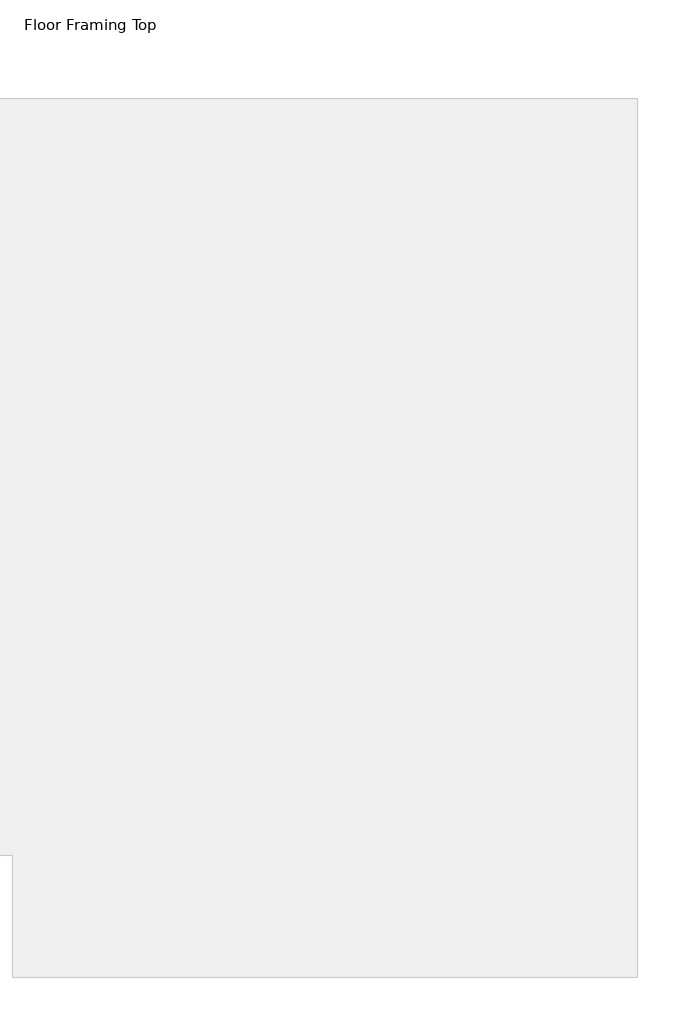
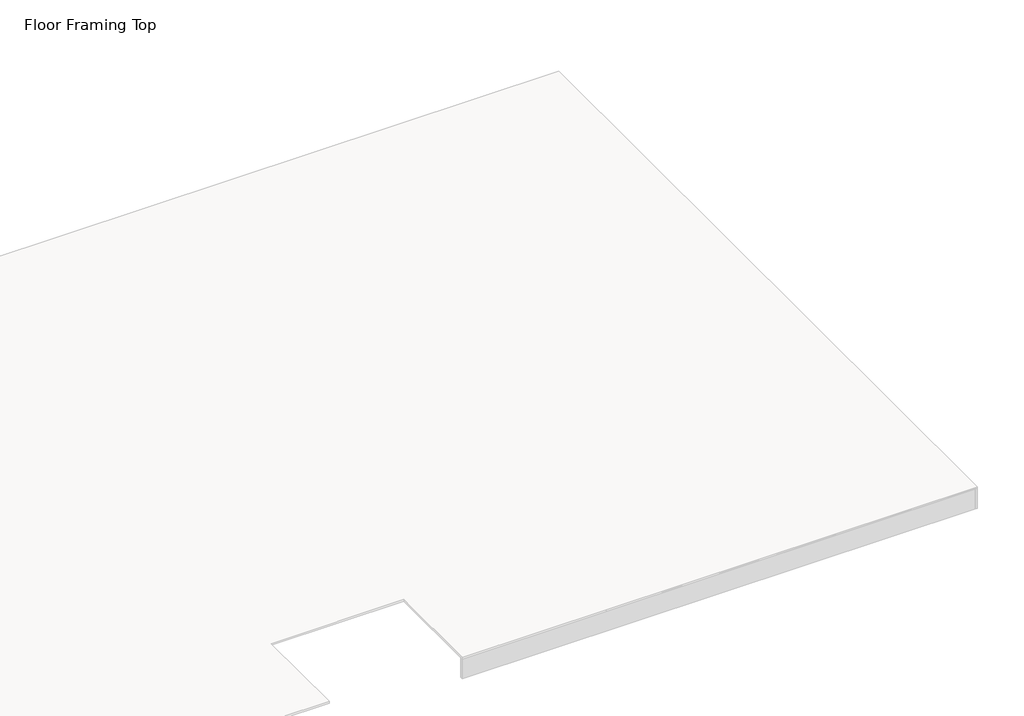
# One storey, part 3 of 4: 17 beams.
"""IFC4 building model written with IfcOpenShell, lengths in millimetres."""

from ifc_helpers import new_model, si_unit, frame, origin, place, context, project, spatial, polyline, outline, extrude, element, save

model = new_model("IFC4")

# Units and contexts
model_context = context("Model", 3, world=origin())
ifc_project = project(units=[si_unit("LENGTHUNIT", "METRE", prefix="MILLI")], contexts=[model_context])

# Site, building, storey
site = spatial("IfcSite", under=ifc_project)
building = spatial("IfcBuilding", under=site)
storey = spatial("IfcBuildingStorey", under=building, Name="Floor Framing Top", Elevation=0.0)

# Beams
placement = place(None, origin())
element("IfcBeam", 1, ObjectType="Plywood Web Joist : 11 7/8 TJI 150", at=placement, inside=storey, context=model_context, shape_type="SweptSolid", body=[
    extrude(outline(polyline([(12853.5472749, -5717.8040947), (12844.0222749, -5717.8040947), (12844.0222749, 4456.4834053), (12853.5472749, 4456.4834053), (12853.5472749, -5717.8040947)])), frame((0.0, 0.0, -269.1410374), z_axis=(0.0, 0.0, 1.0), x_axis=(1.0, 0.0, 0.0)), (0.0, 0.0, 1.0), 237.3910374),
    extrude(outline(polyline([(12844.0222749, -663.2040947), (12844.0222749, 4456.4834053), (12853.5472749, 4456.4834053), (12853.5472749, -663.2040947), (12844.0222749, -663.2040947)])), frame((0.0, 0.0, -269.1410374), z_axis=(0.0, 0.0, 1.0), x_axis=(1.0, 0.0, 0.0)), (0.0, 0.0, 1.0), 237.3910374),
    extrude(outline(polyline([(0.0, 12829.7347749), (-38.1, 12829.7347749), (-38.1, 12844.0222749), (-31.75, 12844.0222749), (-31.75, 12853.5472749), (-38.1, 12853.5472749), (-38.1, 12867.8347749), (0.0, 12867.8347749), (0.0, 12829.7347749)])), frame((0.0, -5717.8040947, 0.0), z_axis=(0.0, 1.0, 0.0), x_axis=(0.0, 0.0, 1.0)), (0.0, 0.0, 1.0), 10174.2875),
    extrude(outline(polyline([(-263.525, 12867.8347749), (-263.525, 12853.5472749), (-269.1410374, 12853.5472749), (-269.1410374, 12844.0222749), (-263.525, 12844.0222749), (-263.525, 12829.7347749), (-301.625, 12829.7347749), (-301.625, 12867.8347749), (-263.525, 12867.8347749)])), frame((0.0, -5717.8040947, 0.0), z_axis=(0.0, 1.0, 0.0), x_axis=(0.0, 0.0, 1.0)), (0.0, 0.0, 1.0), 10174.2875),
    extrude(outline(polyline([(0.0, 12829.7347749), (-38.1, 12829.7347749), (-38.1, 12844.0222749), (-31.75, 12844.0222749), (-31.75, 12853.5472749), (-38.1, 12853.5472749), (-38.1, 12867.8347749), (0.0, 12867.8347749), (0.0, 12829.7347749)])), frame((0.0, -663.2040947, 0.0), z_axis=(0.0, 1.0, 0.0), x_axis=(0.0, 0.0, 1.0)), (0.0, 0.0, 1.0), 5119.6875),
    extrude(outline(polyline([(-263.525, 12867.8347749), (-263.525, 12853.5472749), (-269.1410374, 12853.5472749), (-269.1410374, 12844.0222749), (-263.525, 12844.0222749), (-263.525, 12829.7347749), (-301.625, 12829.7347749), (-301.625, 12867.8347749), (-263.525, 12867.8347749)])), frame((0.0, -663.2040947, 0.0), z_axis=(0.0, 1.0, 0.0), x_axis=(0.0, 0.0, 1.0)), (0.0, 0.0, 1.0), 5119.6875),
])
element("IfcBeam", 2, ObjectType="Plywood Web Joist : 11 7/8 TJI 150", at=placement, inside=storey, context=model_context, shape_type="SweptSolid", body=[
    extrude(outline(polyline([(12447.1472749, -5717.8040947), (12437.6222749, -5717.8040947), (12437.6222749, 4456.4834053), (12447.1472749, 4456.4834053), (12447.1472749, -5717.8040947)])), frame((0.0, 0.0, -269.1410374), z_axis=(0.0, 0.0, 1.0), x_axis=(1.0, 0.0, 0.0)), (0.0, 0.0, 1.0), 237.3910374),
    extrude(outline(polyline([(12437.6222749, -663.2040947), (12437.6222749, 4456.4834053), (12447.1472749, 4456.4834053), (12447.1472749, -663.2040947), (12437.6222749, -663.2040947)])), frame((0.0, 0.0, -269.1410374), z_axis=(0.0, 0.0, 1.0), x_axis=(1.0, 0.0, 0.0)), (0.0, 0.0, 1.0), 237.3910374),
    extrude(outline(polyline([(0.0, 12423.3347749), (-38.1, 12423.3347749), (-38.1, 12437.6222749), (-31.75, 12437.6222749), (-31.75, 12447.1472749), (-38.1, 12447.1472749), (-38.1, 12461.4347749), (0.0, 12461.4347749), (0.0, 12423.3347749)])), frame((0.0, -5717.8040947, 0.0), z_axis=(0.0, 1.0, 0.0), x_axis=(0.0, 0.0, 1.0)), (0.0, 0.0, 1.0), 10174.2875),
    extrude(outline(polyline([(-263.525, 12461.4347749), (-263.525, 12447.1472749), (-269.1410374, 12447.1472749), (-269.1410374, 12437.6222749), (-263.525, 12437.6222749), (-263.525, 12423.3347749), (-301.625, 12423.3347749), (-301.625, 12461.4347749), (-263.525, 12461.4347749)])), frame((0.0, -5717.8040947, 0.0), z_axis=(0.0, 1.0, 0.0), x_axis=(0.0, 0.0, 1.0)), (0.0, 0.0, 1.0), 10174.2875),
    extrude(outline(polyline([(0.0, 12423.3347749), (-38.1, 12423.3347749), (-38.1, 12437.6222749), (-31.75, 12437.6222749), (-31.75, 12447.1472749), (-38.1, 12447.1472749), (-38.1, 12461.4347749), (0.0, 12461.4347749), (0.0, 12423.3347749)])), frame((0.0, -663.2040947, 0.0), z_axis=(0.0, 1.0, 0.0), x_axis=(0.0, 0.0, 1.0)), (0.0, 0.0, 1.0), 5119.6875),
    extrude(outline(polyline([(-263.525, 12461.4347749), (-263.525, 12447.1472749), (-269.1410374, 12447.1472749), (-269.1410374, 12437.6222749), (-263.525, 12437.6222749), (-263.525, 12423.3347749), (-301.625, 12423.3347749), (-301.625, 12461.4347749), (-263.525, 12461.4347749)])), frame((0.0, -663.2040947, 0.0), z_axis=(0.0, 1.0, 0.0), x_axis=(0.0, 0.0, 1.0)), (0.0, 0.0, 1.0), 5119.6875),
])
element("IfcBeam", 3, ObjectType="Plywood Web Joist : 11 7/8 TJI 150", at=placement, inside=storey, context=model_context, shape_type="SweptSolid", body=[
    extrude(outline(polyline([(11634.3472749, -5717.8040947), (11624.8222749, -5717.8040947), (11624.8222749, 4456.4834053), (11634.3472749, 4456.4834053), (11634.3472749, -5717.8040947)])), frame((0.0, 0.0, -269.1410374), z_axis=(0.0, 0.0, 1.0), x_axis=(1.0, 0.0, 0.0)), (0.0, 0.0, 1.0), 237.3910374),
    extrude(outline(polyline([(11624.8222749, -663.2040947), (11624.8222749, 4456.4834053), (11634.3472749, 4456.4834053), (11634.3472749, -663.2040947), (11624.8222749, -663.2040947)])), frame((0.0, 0.0, -269.1410374), z_axis=(0.0, 0.0, 1.0), x_axis=(1.0, 0.0, 0.0)), (0.0, 0.0, 1.0), 237.3910374),
    extrude(outline(polyline([(0.0, 11610.5347749), (-38.1, 11610.5347749), (-38.1, 11624.8222749), (-31.75, 11624.8222749), (-31.75, 11634.3472749), (-38.1, 11634.3472749), (-38.1, 11648.6347749), (0.0, 11648.6347749), (0.0, 11610.5347749)])), frame((0.0, -5717.8040947, 0.0), z_axis=(0.0, 1.0, 0.0), x_axis=(0.0, 0.0, 1.0)), (0.0, 0.0, 1.0), 10174.2875),
    extrude(outline(polyline([(-263.525, 11648.6347749), (-263.525, 11634.3472749), (-269.1410374, 11634.3472749), (-269.1410374, 11624.8222749), (-263.525, 11624.8222749), (-263.525, 11610.5347749), (-301.625, 11610.5347749), (-301.625, 11648.6347749), (-263.525, 11648.6347749)])), frame((0.0, -5717.8040947, 0.0), z_axis=(0.0, 1.0, 0.0), x_axis=(0.0, 0.0, 1.0)), (0.0, 0.0, 1.0), 10174.2875),
    extrude(outline(polyline([(0.0, 11610.5347749), (-38.1, 11610.5347749), (-38.1, 11624.8222749), (-31.75, 11624.8222749), (-31.75, 11634.3472749), (-38.1, 11634.3472749), (-38.1, 11648.6347749), (0.0, 11648.6347749), (0.0, 11610.5347749)])), frame((0.0, -663.2040947, 0.0), z_axis=(0.0, 1.0, 0.0), x_axis=(0.0, 0.0, 1.0)), (0.0, 0.0, 1.0), 5119.6875),
    extrude(outline(polyline([(-263.525, 11648.6347749), (-263.525, 11634.3472749), (-269.1410374, 11634.3472749), (-269.1410374, 11624.8222749), (-263.525, 11624.8222749), (-263.525, 11610.5347749), (-301.625, 11610.5347749), (-301.625, 11648.6347749), (-263.525, 11648.6347749)])), frame((0.0, -663.2040947, 0.0), z_axis=(0.0, 1.0, 0.0), x_axis=(0.0, 0.0, 1.0)), (0.0, 0.0, 1.0), 5119.6875),
])
element("IfcBeam", 4, ObjectType="Plywood Web Joist : 11 7/8 TJI 150", at=placement, inside=storey, context=model_context, shape_type="SweptSolid", body=[
    extrude(outline(polyline([(11227.9472749, -5717.8040947), (11218.4222749, -5717.8040947), (11218.4222749, 4456.4834053), (11227.9472749, 4456.4834053), (11227.9472749, -5717.8040947)])), frame((0.0, 0.0, -269.1410374), z_axis=(0.0, 0.0, 1.0), x_axis=(1.0, 0.0, 0.0)), (0.0, 0.0, 1.0), 237.3910374),
    extrude(outline(polyline([(11218.4222749, -663.2040947), (11218.4222749, 4456.4834053), (11227.9472749, 4456.4834053), (11227.9472749, -663.2040947), (11218.4222749, -663.2040947)])), frame((0.0, 0.0, -269.1410374), z_axis=(0.0, 0.0, 1.0), x_axis=(1.0, 0.0, 0.0)), (0.0, 0.0, 1.0), 237.3910374),
    extrude(outline(polyline([(0.0, 11204.1347749), (-38.1, 11204.1347749), (-38.1, 11218.4222749), (-31.75, 11218.4222749), (-31.75, 11227.9472749), (-38.1, 11227.9472749), (-38.1, 11242.2347749), (0.0, 11242.2347749), (0.0, 11204.1347749)])), frame((0.0, -5717.8040947, 0.0), z_axis=(0.0, 1.0, 0.0), x_axis=(0.0, 0.0, 1.0)), (0.0, 0.0, 1.0), 10174.2875),
    extrude(outline(polyline([(-263.525, 11242.2347749), (-263.525, 11227.9472749), (-269.1410374, 11227.9472749), (-269.1410374, 11218.4222749), (-263.525, 11218.4222749), (-263.525, 11204.1347749), (-301.625, 11204.1347749), (-301.625, 11242.2347749), (-263.525, 11242.2347749)])), frame((0.0, -5717.8040947, 0.0), z_axis=(0.0, 1.0, 0.0), x_axis=(0.0, 0.0, 1.0)), (0.0, 0.0, 1.0), 10174.2875),
    extrude(outline(polyline([(0.0, 11204.1347749), (-38.1, 11204.1347749), (-38.1, 11218.4222749), (-31.75, 11218.4222749), (-31.75, 11227.9472749), (-38.1, 11227.9472749), (-38.1, 11242.2347749), (0.0, 11242.2347749), (0.0, 11204.1347749)])), frame((0.0, -663.2040947, 0.0), z_axis=(0.0, 1.0, 0.0), x_axis=(0.0, 0.0, 1.0)), (0.0, 0.0, 1.0), 5119.6875),
    extrude(outline(polyline([(-263.525, 11242.2347749), (-263.525, 11227.9472749), (-269.1410374, 11227.9472749), (-269.1410374, 11218.4222749), (-263.525, 11218.4222749), (-263.525, 11204.1347749), (-301.625, 11204.1347749), (-301.625, 11242.2347749), (-263.525, 11242.2347749)])), frame((0.0, -663.2040947, 0.0), z_axis=(0.0, 1.0, 0.0), x_axis=(0.0, 0.0, 1.0)), (0.0, 0.0, 1.0), 5119.6875),
])
element("IfcBeam", 5, ObjectType="Plywood Web Joist : 11 7/8 TJI 150", at=placement, inside=storey, context=model_context, shape_type="SweptSolid", body=[
    extrude(outline(polyline([(10821.5472749, -5717.8040947), (10812.0222749, -5717.8040947), (10812.0222749, 4456.4834053), (10821.5472749, 4456.4834053), (10821.5472749, -5717.8040947)])), frame((0.0, 0.0, -269.1410374), z_axis=(0.0, 0.0, 1.0), x_axis=(1.0, 0.0, 0.0)), (0.0, 0.0, 1.0), 237.3910374),
    extrude(outline(polyline([(10812.0222749, -663.2040947), (10812.0222749, 4456.4834053), (10821.5472749, 4456.4834053), (10821.5472749, -663.2040947), (10812.0222749, -663.2040947)])), frame((0.0, 0.0, -269.1410374), z_axis=(0.0, 0.0, 1.0), x_axis=(1.0, 0.0, 0.0)), (0.0, 0.0, 1.0), 237.3910374),
    extrude(outline(polyline([(0.0, 10797.7347749), (-38.1, 10797.7347749), (-38.1, 10812.0222749), (-31.75, 10812.0222749), (-31.75, 10821.5472749), (-38.1, 10821.5472749), (-38.1, 10835.8347749), (0.0, 10835.8347749), (0.0, 10797.7347749)])), frame((0.0, -5717.8040947, 0.0), z_axis=(0.0, 1.0, 0.0), x_axis=(0.0, 0.0, 1.0)), (0.0, 0.0, 1.0), 10174.2875),
    extrude(outline(polyline([(-263.525, 10835.8347749), (-263.525, 10821.5472749), (-269.1410374, 10821.5472749), (-269.1410374, 10812.0222749), (-263.525, 10812.0222749), (-263.525, 10797.7347749), (-301.625, 10797.7347749), (-301.625, 10835.8347749), (-263.525, 10835.8347749)])), frame((0.0, -5717.8040947, 0.0), z_axis=(0.0, 1.0, 0.0), x_axis=(0.0, 0.0, 1.0)), (0.0, 0.0, 1.0), 10174.2875),
    extrude(outline(polyline([(0.0, 10797.7347749), (-38.1, 10797.7347749), (-38.1, 10812.0222749), (-31.75, 10812.0222749), (-31.75, 10821.5472749), (-38.1, 10821.5472749), (-38.1, 10835.8347749), (0.0, 10835.8347749), (0.0, 10797.7347749)])), frame((0.0, -663.2040947, 0.0), z_axis=(0.0, 1.0, 0.0), x_axis=(0.0, 0.0, 1.0)), (0.0, 0.0, 1.0), 5119.6875),
    extrude(outline(polyline([(-263.525, 10835.8347749), (-263.525, 10821.5472749), (-269.1410374, 10821.5472749), (-269.1410374, 10812.0222749), (-263.525, 10812.0222749), (-263.525, 10797.7347749), (-301.625, 10797.7347749), (-301.625, 10835.8347749), (-263.525, 10835.8347749)])), frame((0.0, -663.2040947, 0.0), z_axis=(0.0, 1.0, 0.0), x_axis=(0.0, 0.0, 1.0)), (0.0, 0.0, 1.0), 5119.6875),
])
element("IfcBeam", 6, ObjectType="Plywood Web Joist : 11 7/8 TJI 150", at=placement, inside=storey, context=model_context, shape_type="SweptSolid", body=[
    extrude(outline(polyline([(10415.1472749, -5717.8040947), (10405.6222749, -5717.8040947), (10405.6222749, 4456.4834053), (10415.1472749, 4456.4834053), (10415.1472749, -5717.8040947)])), frame((0.0, 0.0, -269.1410374), z_axis=(0.0, 0.0, 1.0), x_axis=(1.0, 0.0, 0.0)), (0.0, 0.0, 1.0), 237.3910374),
    extrude(outline(polyline([(10405.6222749, -663.2040947), (10405.6222749, 4456.4834053), (10415.1472749, 4456.4834053), (10415.1472749, -663.2040947), (10405.6222749, -663.2040947)])), frame((0.0, 0.0, -269.1410374), z_axis=(0.0, 0.0, 1.0), x_axis=(1.0, 0.0, 0.0)), (0.0, 0.0, 1.0), 237.3910374),
    extrude(outline(polyline([(0.0, 10391.3347749), (-38.1, 10391.3347749), (-38.1, 10405.6222749), (-31.75, 10405.6222749), (-31.75, 10415.1472749), (-38.1, 10415.1472749), (-38.1, 10429.4347749), (0.0, 10429.4347749), (0.0, 10391.3347749)])), frame((0.0, -5717.8040947, 0.0), z_axis=(0.0, 1.0, 0.0), x_axis=(0.0, 0.0, 1.0)), (0.0, 0.0, 1.0), 10174.2875),
    extrude(outline(polyline([(-263.525, 10429.4347749), (-263.525, 10415.1472749), (-269.1410374, 10415.1472749), (-269.1410374, 10405.6222749), (-263.525, 10405.6222749), (-263.525, 10391.3347749), (-301.625, 10391.3347749), (-301.625, 10429.4347749), (-263.525, 10429.4347749)])), frame((0.0, -5717.8040947, 0.0), z_axis=(0.0, 1.0, 0.0), x_axis=(0.0, 0.0, 1.0)), (0.0, 0.0, 1.0), 10174.2875),
    extrude(outline(polyline([(0.0, 10391.3347749), (-38.1, 10391.3347749), (-38.1, 10405.6222749), (-31.75, 10405.6222749), (-31.75, 10415.1472749), (-38.1, 10415.1472749), (-38.1, 10429.4347749), (0.0, 10429.4347749), (0.0, 10391.3347749)])), frame((0.0, -663.2040947, 0.0), z_axis=(0.0, 1.0, 0.0), x_axis=(0.0, 0.0, 1.0)), (0.0, 0.0, 1.0), 5119.6875),
    extrude(outline(polyline([(-263.525, 10429.4347749), (-263.525, 10415.1472749), (-269.1410374, 10415.1472749), (-269.1410374, 10405.6222749), (-263.525, 10405.6222749), (-263.525, 10391.3347749), (-301.625, 10391.3347749), (-301.625, 10429.4347749), (-263.525, 10429.4347749)])), frame((0.0, -663.2040947, 0.0), z_axis=(0.0, 1.0, 0.0), x_axis=(0.0, 0.0, 1.0)), (0.0, 0.0, 1.0), 5119.6875),
])
element("IfcBeam", 7, ObjectType="Plywood Web Joist : 11 7/8 TJI 150", at=placement, inside=storey, context=model_context, shape_type="SweptSolid", body=[
    extrude(outline(polyline([(10008.7472749, -5717.8040947), (9999.2222749, -5717.8040947), (9999.2222749, 4456.4834053), (10008.7472749, 4456.4834053), (10008.7472749, -5717.8040947)])), frame((0.0, 0.0, -269.1410374), z_axis=(0.0, 0.0, 1.0), x_axis=(1.0, 0.0, 0.0)), (0.0, 0.0, 1.0), 237.3910374),
    extrude(outline(polyline([(9999.2222749, -663.2040947), (9999.2222749, 4456.4834053), (10008.7472749, 4456.4834053), (10008.7472749, -663.2040947), (9999.2222749, -663.2040947)])), frame((0.0, 0.0, -269.1410374), z_axis=(0.0, 0.0, 1.0), x_axis=(1.0, 0.0, 0.0)), (0.0, 0.0, 1.0), 237.3910374),
    extrude(outline(polyline([(0.0, 9984.9347749), (-38.1, 9984.9347749), (-38.1, 9999.2222749), (-31.75, 9999.2222749), (-31.75, 10008.7472749), (-38.1, 10008.7472749), (-38.1, 10023.0347749), (0.0, 10023.0347749), (0.0, 9984.9347749)])), frame((0.0, -5717.8040947, 0.0), z_axis=(0.0, 1.0, 0.0), x_axis=(0.0, 0.0, 1.0)), (0.0, 0.0, 1.0), 10174.2875),
    extrude(outline(polyline([(-263.525, 10023.0347749), (-263.525, 10008.7472749), (-269.1410374, 10008.7472749), (-269.1410374, 9999.2222749), (-263.525, 9999.2222749), (-263.525, 9984.9347749), (-301.625, 9984.9347749), (-301.625, 10023.0347749), (-263.525, 10023.0347749)])), frame((0.0, -5717.8040947, 0.0), z_axis=(0.0, 1.0, 0.0), x_axis=(0.0, 0.0, 1.0)), (0.0, 0.0, 1.0), 10174.2875),
    extrude(outline(polyline([(0.0, 9984.9347749), (-38.1, 9984.9347749), (-38.1, 9999.2222749), (-31.75, 9999.2222749), (-31.75, 10008.7472749), (-38.1, 10008.7472749), (-38.1, 10023.0347749), (0.0, 10023.0347749), (0.0, 9984.9347749)])), frame((0.0, -663.2040947, 0.0), z_axis=(0.0, 1.0, 0.0), x_axis=(0.0, 0.0, 1.0)), (0.0, 0.0, 1.0), 5119.6875),
    extrude(outline(polyline([(-263.525, 10023.0347749), (-263.525, 10008.7472749), (-269.1410374, 10008.7472749), (-269.1410374, 9999.2222749), (-263.525, 9999.2222749), (-263.525, 9984.9347749), (-301.625, 9984.9347749), (-301.625, 10023.0347749), (-263.525, 10023.0347749)])), frame((0.0, -663.2040947, 0.0), z_axis=(0.0, 1.0, 0.0), x_axis=(0.0, 0.0, 1.0)), (0.0, 0.0, 1.0), 5119.6875),
])
element("IfcBeam", 8, ObjectType="Plywood Web Joist : 11 7/8 TJI 150", at=placement, inside=storey, context=model_context, shape_type="SweptSolid", body=[
    extrude(outline(polyline([(9602.3472749, -5717.8040947), (9592.8222749, -5717.8040947), (9592.8222749, 4456.4834053), (9602.3472749, 4456.4834053), (9602.3472749, -5717.8040947)])), frame((0.0, 0.0, -269.1410374), z_axis=(0.0, 0.0, 1.0), x_axis=(1.0, 0.0, 0.0)), (0.0, 0.0, 1.0), 237.3910374),
    extrude(outline(polyline([(9592.8222749, -663.2040947), (9592.8222749, 4456.4834053), (9602.3472749, 4456.4834053), (9602.3472749, -663.2040947), (9592.8222749, -663.2040947)])), frame((0.0, 0.0, -269.1410374), z_axis=(0.0, 0.0, 1.0), x_axis=(1.0, 0.0, 0.0)), (0.0, 0.0, 1.0), 237.3910374),
    extrude(outline(polyline([(0.0, 9578.5347749), (-38.1, 9578.5347749), (-38.1, 9592.8222749), (-31.75, 9592.8222749), (-31.75, 9602.3472749), (-38.1, 9602.3472749), (-38.1, 9616.6347749), (0.0, 9616.6347749), (0.0, 9578.5347749)])), frame((0.0, -5717.8040947, 0.0), z_axis=(0.0, 1.0, 0.0), x_axis=(0.0, 0.0, 1.0)), (0.0, 0.0, 1.0), 10174.2875),
    extrude(outline(polyline([(-263.525, 9616.6347749), (-263.525, 9602.3472749), (-269.1410374, 9602.3472749), (-269.1410374, 9592.8222749), (-263.525, 9592.8222749), (-263.525, 9578.5347749), (-301.625, 9578.5347749), (-301.625, 9616.6347749), (-263.525, 9616.6347749)])), frame((0.0, -5717.8040947, 0.0), z_axis=(0.0, 1.0, 0.0), x_axis=(0.0, 0.0, 1.0)), (0.0, 0.0, 1.0), 10174.2875),
    extrude(outline(polyline([(0.0, 9578.5347749), (-38.1, 9578.5347749), (-38.1, 9592.8222749), (-31.75, 9592.8222749), (-31.75, 9602.3472749), (-38.1, 9602.3472749), (-38.1, 9616.6347749), (0.0, 9616.6347749), (0.0, 9578.5347749)])), frame((0.0, -663.2040947, 0.0), z_axis=(0.0, 1.0, 0.0), x_axis=(0.0, 0.0, 1.0)), (0.0, 0.0, 1.0), 5119.6875),
    extrude(outline(polyline([(-263.525, 9616.6347749), (-263.525, 9602.3472749), (-269.1410374, 9602.3472749), (-269.1410374, 9592.8222749), (-263.525, 9592.8222749), (-263.525, 9578.5347749), (-301.625, 9578.5347749), (-301.625, 9616.6347749), (-263.525, 9616.6347749)])), frame((0.0, -663.2040947, 0.0), z_axis=(0.0, 1.0, 0.0), x_axis=(0.0, 0.0, 1.0)), (0.0, 0.0, 1.0), 5119.6875),
])
element("IfcBeam", 9, ObjectType="Plywood Web Joist : 11 7/8 TJI 150", at=placement, inside=storey, context=model_context, shape_type="SweptSolid", body=[
    extrude(outline(polyline([(9195.9472749, -5717.8040947), (9186.4222749, -5717.8040947), (9186.4222749, 4456.4834053), (9195.9472749, 4456.4834053), (9195.9472749, -5717.8040947)])), frame((0.0, 0.0, -269.1410374), z_axis=(0.0, 0.0, 1.0), x_axis=(1.0, 0.0, 0.0)), (0.0, 0.0, 1.0), 237.3910374),
    extrude(outline(polyline([(9186.4222749, -663.2040947), (9186.4222749, 4456.4834053), (9195.9472749, 4456.4834053), (9195.9472749, -663.2040947), (9186.4222749, -663.2040947)])), frame((0.0, 0.0, -269.1410374), z_axis=(0.0, 0.0, 1.0), x_axis=(1.0, 0.0, 0.0)), (0.0, 0.0, 1.0), 237.3910374),
    extrude(outline(polyline([(0.0, 9172.1347749), (-38.1, 9172.1347749), (-38.1, 9186.4222749), (-31.75, 9186.4222749), (-31.75, 9195.9472749), (-38.1, 9195.9472749), (-38.1, 9210.2347749), (0.0, 9210.2347749), (0.0, 9172.1347749)])), frame((0.0, -5717.8040947, 0.0), z_axis=(0.0, 1.0, 0.0), x_axis=(0.0, 0.0, 1.0)), (0.0, 0.0, 1.0), 10174.2875),
    extrude(outline(polyline([(-263.525, 9210.2347749), (-263.525, 9195.9472749), (-269.1410374, 9195.9472749), (-269.1410374, 9186.4222749), (-263.525, 9186.4222749), (-263.525, 9172.1347749), (-301.625, 9172.1347749), (-301.625, 9210.2347749), (-263.525, 9210.2347749)])), frame((0.0, -5717.8040947, 0.0), z_axis=(0.0, 1.0, 0.0), x_axis=(0.0, 0.0, 1.0)), (0.0, 0.0, 1.0), 10174.2875),
    extrude(outline(polyline([(0.0, 9172.1347749), (-38.1, 9172.1347749), (-38.1, 9186.4222749), (-31.75, 9186.4222749), (-31.75, 9195.9472749), (-38.1, 9195.9472749), (-38.1, 9210.2347749), (0.0, 9210.2347749), (0.0, 9172.1347749)])), frame((0.0, -663.2040947, 0.0), z_axis=(0.0, 1.0, 0.0), x_axis=(0.0, 0.0, 1.0)), (0.0, 0.0, 1.0), 5119.6875),
    extrude(outline(polyline([(-263.525, 9210.2347749), (-263.525, 9195.9472749), (-269.1410374, 9195.9472749), (-269.1410374, 9186.4222749), (-263.525, 9186.4222749), (-263.525, 9172.1347749), (-301.625, 9172.1347749), (-301.625, 9210.2347749), (-263.525, 9210.2347749)])), frame((0.0, -663.2040947, 0.0), z_axis=(0.0, 1.0, 0.0), x_axis=(0.0, 0.0, 1.0)), (0.0, 0.0, 1.0), 5119.6875),
])
element("IfcBeam", 10, ObjectType="Plywood Web Joist : 11 7/8 TJI 150", at=placement, inside=storey, context=model_context, shape_type="SweptSolid", body=[
    extrude(outline(polyline([(8789.5472749, -5717.8040947), (8780.0222749, -5717.8040947), (8780.0222749, 4456.4834053), (8789.5472749, 4456.4834053), (8789.5472749, -5717.8040947)])), frame((0.0, 0.0, -269.1410374), z_axis=(0.0, 0.0, 1.0), x_axis=(1.0, 0.0, 0.0)), (0.0, 0.0, 1.0), 237.3910374),
    extrude(outline(polyline([(8780.0222749, -663.2040947), (8780.0222749, 4456.4834053), (8789.5472749, 4456.4834053), (8789.5472749, -663.2040947), (8780.0222749, -663.2040947)])), frame((0.0, 0.0, -269.1410374), z_axis=(0.0, 0.0, 1.0), x_axis=(1.0, 0.0, 0.0)), (0.0, 0.0, 1.0), 237.3910374),
    extrude(outline(polyline([(0.0, 8765.7347749), (-38.1, 8765.7347749), (-38.1, 8780.0222749), (-31.75, 8780.0222749), (-31.75, 8789.5472749), (-38.1, 8789.5472749), (-38.1, 8803.8347749), (0.0, 8803.8347749), (0.0, 8765.7347749)])), frame((0.0, -5717.8040947, 0.0), z_axis=(0.0, 1.0, 0.0), x_axis=(0.0, 0.0, 1.0)), (0.0, 0.0, 1.0), 10174.2875),
    extrude(outline(polyline([(-263.525, 8803.8347749), (-263.525, 8789.5472749), (-269.1410374, 8789.5472749), (-269.1410374, 8780.0222749), (-263.525, 8780.0222749), (-263.525, 8765.7347749), (-301.625, 8765.7347749), (-301.625, 8803.8347749), (-263.525, 8803.8347749)])), frame((0.0, -5717.8040947, 0.0), z_axis=(0.0, 1.0, 0.0), x_axis=(0.0, 0.0, 1.0)), (0.0, 0.0, 1.0), 10174.2875),
    extrude(outline(polyline([(0.0, 8765.7347749), (-38.1, 8765.7347749), (-38.1, 8780.0222749), (-31.75, 8780.0222749), (-31.75, 8789.5472749), (-38.1, 8789.5472749), (-38.1, 8803.8347749), (0.0, 8803.8347749), (0.0, 8765.7347749)])), frame((0.0, -663.2040947, 0.0), z_axis=(0.0, 1.0, 0.0), x_axis=(0.0, 0.0, 1.0)), (0.0, 0.0, 1.0), 5119.6875),
    extrude(outline(polyline([(-263.525, 8803.8347749), (-263.525, 8789.5472749), (-269.1410374, 8789.5472749), (-269.1410374, 8780.0222749), (-263.525, 8780.0222749), (-263.525, 8765.7347749), (-301.625, 8765.7347749), (-301.625, 8803.8347749), (-263.525, 8803.8347749)])), frame((0.0, -663.2040947, 0.0), z_axis=(0.0, 1.0, 0.0), x_axis=(0.0, 0.0, 1.0)), (0.0, 0.0, 1.0), 5119.6875),
])
element("IfcBeam", 11, ObjectType="Plywood Web Joist : 11 7/8 TJI 150", at=placement, inside=storey, context=model_context, shape_type="SweptSolid", body=[
    extrude(outline(polyline([(8383.1472749, -5717.8040947), (8373.6222749, -5717.8040947), (8373.6222749, 4456.4834053), (8383.1472749, 4456.4834053), (8383.1472749, -5717.8040947)])), frame((0.0, 0.0, -269.1410374), z_axis=(0.0, 0.0, 1.0), x_axis=(1.0, 0.0, 0.0)), (0.0, 0.0, 1.0), 237.3910374),
    extrude(outline(polyline([(8373.6222749, -663.2040947), (8373.6222749, 4456.4834053), (8383.1472749, 4456.4834053), (8383.1472749, -663.2040947), (8373.6222749, -663.2040947)])), frame((0.0, 0.0, -269.1410374), z_axis=(0.0, 0.0, 1.0), x_axis=(1.0, 0.0, 0.0)), (0.0, 0.0, 1.0), 237.3910374),
    extrude(outline(polyline([(0.0, 8359.3347749), (-38.1, 8359.3347749), (-38.1, 8373.6222749), (-31.75, 8373.6222749), (-31.75, 8383.1472749), (-38.1, 8383.1472749), (-38.1, 8397.4347749), (0.0, 8397.4347749), (0.0, 8359.3347749)])), frame((0.0, -5717.8040947, 0.0), z_axis=(0.0, 1.0, 0.0), x_axis=(0.0, 0.0, 1.0)), (0.0, 0.0, 1.0), 10174.2875),
    extrude(outline(polyline([(-263.525, 8397.4347749), (-263.525, 8383.1472749), (-269.1410374, 8383.1472749), (-269.1410374, 8373.6222749), (-263.525, 8373.6222749), (-263.525, 8359.3347749), (-301.625, 8359.3347749), (-301.625, 8397.4347749), (-263.525, 8397.4347749)])), frame((0.0, -5717.8040947, 0.0), z_axis=(0.0, 1.0, 0.0), x_axis=(0.0, 0.0, 1.0)), (0.0, 0.0, 1.0), 10174.2875),
    extrude(outline(polyline([(0.0, 8359.3347749), (-38.1, 8359.3347749), (-38.1, 8373.6222749), (-31.75, 8373.6222749), (-31.75, 8383.1472749), (-38.1, 8383.1472749), (-38.1, 8397.4347749), (0.0, 8397.4347749), (0.0, 8359.3347749)])), frame((0.0, -663.2040947, 0.0), z_axis=(0.0, 1.0, 0.0), x_axis=(0.0, 0.0, 1.0)), (0.0, 0.0, 1.0), 5119.6875),
    extrude(outline(polyline([(-263.525, 8397.4347749), (-263.525, 8383.1472749), (-269.1410374, 8383.1472749), (-269.1410374, 8373.6222749), (-263.525, 8373.6222749), (-263.525, 8359.3347749), (-301.625, 8359.3347749), (-301.625, 8397.4347749), (-263.525, 8397.4347749)])), frame((0.0, -663.2040947, 0.0), z_axis=(0.0, 1.0, 0.0), x_axis=(0.0, 0.0, 1.0)), (0.0, 0.0, 1.0), 5119.6875),
])
element("IfcBeam", 12, ObjectType="Plywood Web Joist : 11 7/8 TJI 150", at=placement, inside=storey, context=model_context, shape_type="SweptSolid", body=[
    extrude(outline(polyline([(10821.5472749, -701.3040947), (10821.5472749, -5717.8040947), (10812.0222749, -5717.8040947), (10812.0222749, -701.3040947), (10821.5472749, -701.3040947)])), frame((0.0, 0.0, -269.1410374), z_axis=(0.0, 0.0, 1.0), x_axis=(1.0, 0.0, 0.0)), (0.0, 0.0, 1.0), 237.3910374),
    extrude(outline(polyline([(0.0, 10797.7347749), (-38.1, 10797.7347749), (-38.1, 10812.0222749), (-31.75, 10812.0222749), (-31.75, 10821.5472749), (-38.1, 10821.5472749), (-38.1, 10835.8347749), (0.0, 10835.8347749), (0.0, 10797.7347749)])), frame((0.0, -5717.8040947, 0.0), z_axis=(0.0, 1.0, 0.0), x_axis=(0.0, 0.0, 1.0)), (0.0, 0.0, 1.0), 5016.5),
    extrude(outline(polyline([(-263.525, 10835.8347749), (-263.525, 10821.5472749), (-269.1410374, 10821.5472749), (-269.1410374, 10812.0222749), (-263.525, 10812.0222749), (-263.525, 10797.7347749), (-301.625, 10797.7347749), (-301.625, 10835.8347749), (-263.525, 10835.8347749)])), frame((0.0, -5717.8040947, 0.0), z_axis=(0.0, 1.0, 0.0), x_axis=(0.0, 0.0, 1.0)), (0.0, 0.0, 1.0), 5016.5),
])
element("IfcBeam", 13, ObjectType="Plywood Web Joist : 11 7/8 TJI 150", at=placement, inside=storey, context=model_context, shape_type="SweptSolid", body=[
    extrude(outline(polyline([(11227.9472749, -701.3040947), (11227.9472749, -5717.8040947), (11218.4222749, -5717.8040947), (11218.4222749, -701.3040947), (11227.9472749, -701.3040947)])), frame((0.0, 0.0, -269.1410374), z_axis=(0.0, 0.0, 1.0), x_axis=(1.0, 0.0, 0.0)), (0.0, 0.0, 1.0), 237.3910374),
    extrude(outline(polyline([(0.0, 11204.1347749), (-38.1, 11204.1347749), (-38.1, 11218.4222749), (-31.75, 11218.4222749), (-31.75, 11227.9472749), (-38.1, 11227.9472749), (-38.1, 11242.2347749), (0.0, 11242.2347749), (0.0, 11204.1347749)])), frame((0.0, -5717.8040947, 0.0), z_axis=(0.0, 1.0, 0.0), x_axis=(0.0, 0.0, 1.0)), (0.0, 0.0, 1.0), 5016.5),
    extrude(outline(polyline([(-263.525, 11242.2347749), (-263.525, 11227.9472749), (-269.1410374, 11227.9472749), (-269.1410374, 11218.4222749), (-263.525, 11218.4222749), (-263.525, 11204.1347749), (-301.625, 11204.1347749), (-301.625, 11242.2347749), (-263.525, 11242.2347749)])), frame((0.0, -5717.8040947, 0.0), z_axis=(0.0, 1.0, 0.0), x_axis=(0.0, 0.0, 1.0)), (0.0, 0.0, 1.0), 5016.5),
])
element("IfcBeam", 14, ObjectType="Plywood Web Joist : 11 7/8 TJI 150", at=placement, inside=storey, context=model_context, shape_type="SweptSolid", body=[
    extrude(outline(polyline([(11634.3472749, -701.3040947), (11634.3472749, -5717.8040947), (11624.8222749, -5717.8040947), (11624.8222749, -701.3040947), (11634.3472749, -701.3040947)])), frame((0.0, 0.0, -269.1410374), z_axis=(0.0, 0.0, 1.0), x_axis=(1.0, 0.0, 0.0)), (0.0, 0.0, 1.0), 237.3910374),
    extrude(outline(polyline([(0.0, 11610.5347749), (-38.1, 11610.5347749), (-38.1, 11624.8222749), (-31.75, 11624.8222749), (-31.75, 11634.3472749), (-38.1, 11634.3472749), (-38.1, 11648.6347749), (0.0, 11648.6347749), (0.0, 11610.5347749)])), frame((0.0, -5717.8040947, 0.0), z_axis=(0.0, 1.0, 0.0), x_axis=(0.0, 0.0, 1.0)), (0.0, 0.0, 1.0), 5016.5),
    extrude(outline(polyline([(-263.525, 11648.6347749), (-263.525, 11634.3472749), (-269.1410374, 11634.3472749), (-269.1410374, 11624.8222749), (-263.525, 11624.8222749), (-263.525, 11610.5347749), (-301.625, 11610.5347749), (-301.625, 11648.6347749), (-263.525, 11648.6347749)])), frame((0.0, -5717.8040947, 0.0), z_axis=(0.0, 1.0, 0.0), x_axis=(0.0, 0.0, 1.0)), (0.0, 0.0, 1.0), 5016.5),
])
element("IfcBeam", 15, ObjectType="Plywood Web Joist : 11 7/8 TJI 150", at=placement, inside=storey, context=model_context, shape_type="SweptSolid", body=[
    extrude(outline(polyline([(12040.7472749, -701.3040947), (12040.7472749, -5717.8040947), (12031.2222749, -5717.8040947), (12031.2222749, -701.3040947), (12040.7472749, -701.3040947)])), frame((0.0, 0.0, -269.1410374), z_axis=(0.0, 0.0, 1.0), x_axis=(1.0, 0.0, 0.0)), (0.0, 0.0, 1.0), 237.3910374),
    extrude(outline(polyline([(0.0, 12016.9347749), (-38.1, 12016.9347749), (-38.1, 12031.2222749), (-31.75, 12031.2222749), (-31.75, 12040.7472749), (-38.1, 12040.7472749), (-38.1, 12055.0347749), (0.0, 12055.0347749), (0.0, 12016.9347749)])), frame((0.0, -5717.8040947, 0.0), z_axis=(0.0, 1.0, 0.0), x_axis=(0.0, 0.0, 1.0)), (0.0, 0.0, 1.0), 5016.5),
    extrude(outline(polyline([(-263.525, 12055.0347749), (-263.525, 12040.7472749), (-269.1410374, 12040.7472749), (-269.1410374, 12031.2222749), (-263.525, 12031.2222749), (-263.525, 12016.9347749), (-301.625, 12016.9347749), (-301.625, 12055.0347749), (-263.525, 12055.0347749)])), frame((0.0, -5717.8040947, 0.0), z_axis=(0.0, 1.0, 0.0), x_axis=(0.0, 0.0, 1.0)), (0.0, 0.0, 1.0), 5016.5),
])
element("IfcBeam", 16, ObjectType="Plywood Web Joist : 11 7/8 TJI 150", at=placement, inside=storey, context=model_context, shape_type="SweptSolid", body=[
    extrude(outline(polyline([(12447.1472749, -701.3040947), (12447.1472749, -5717.8040947), (12437.6222749, -5717.8040947), (12437.6222749, -701.3040947), (12447.1472749, -701.3040947)])), frame((0.0, 0.0, -269.1410374), z_axis=(0.0, 0.0, 1.0), x_axis=(1.0, 0.0, 0.0)), (0.0, 0.0, 1.0), 237.3910374),
    extrude(outline(polyline([(0.0, 12423.3347749), (-38.1, 12423.3347749), (-38.1, 12437.6222749), (-31.75, 12437.6222749), (-31.75, 12447.1472749), (-38.1, 12447.1472749), (-38.1, 12461.4347749), (0.0, 12461.4347749), (0.0, 12423.3347749)])), frame((0.0, -5717.8040947, 0.0), z_axis=(0.0, 1.0, 0.0), x_axis=(0.0, 0.0, 1.0)), (0.0, 0.0, 1.0), 5016.5),
    extrude(outline(polyline([(-263.525, 12461.4347749), (-263.525, 12447.1472749), (-269.1410374, 12447.1472749), (-269.1410374, 12437.6222749), (-263.525, 12437.6222749), (-263.525, 12423.3347749), (-301.625, 12423.3347749), (-301.625, 12461.4347749), (-263.525, 12461.4347749)])), frame((0.0, -5717.8040947, 0.0), z_axis=(0.0, 1.0, 0.0), x_axis=(0.0, 0.0, 1.0)), (0.0, 0.0, 1.0), 5016.5),
])
element("IfcBeam", 17, ObjectType="Plywood Web Joist : 11 7/8 TJI 150", at=placement, inside=storey, context=model_context, shape_type="SweptSolid", body=[
    extrude(outline(polyline([(12853.5472749, -701.3040947), (12853.5472749, -5717.8040947), (12844.0222749, -5717.8040947), (12844.0222749, -701.3040947), (12853.5472749, -701.3040947)])), frame((0.0, 0.0, -269.1410374), z_axis=(0.0, 0.0, 1.0), x_axis=(1.0, 0.0, 0.0)), (0.0, 0.0, 1.0), 237.3910374),
    extrude(outline(polyline([(0.0, 12829.7347749), (-38.1, 12829.7347749), (-38.1, 12844.0222749), (-31.75, 12844.0222749), (-31.75, 12853.5472749), (-38.1, 12853.5472749), (-38.1, 12867.8347749), (0.0, 12867.8347749), (0.0, 12829.7347749)])), frame((0.0, -5717.8040947, 0.0), z_axis=(0.0, 1.0, 0.0), x_axis=(0.0, 0.0, 1.0)), (0.0, 0.0, 1.0), 5016.5),
    extrude(outline(polyline([(-263.525, 12867.8347749), (-263.525, 12853.5472749), (-269.1410374, 12853.5472749), (-269.1410374, 12844.0222749), (-263.525, 12844.0222749), (-263.525, 12829.7347749), (-301.625, 12829.7347749), (-301.625, 12867.8347749), (-263.525, 12867.8347749)])), frame((0.0, -5717.8040947, 0.0), z_axis=(0.0, 1.0, 0.0), x_axis=(0.0, 0.0, 1.0)), (0.0, 0.0, 1.0), 5016.5),
])

save(model, "model.ifc")

# Revit data of these elements
# Type "Plywood Web Joist : 11 7/8 TJI 150"
#   Assembly Code = "B10"
#   Cost = 17.5
#   Length [instance default] = 5' - 0"
#   b = 0' - 1 1/2"
#   d = 0' - 11 7/8"
#   Structural Material [instance default] = Softwood, Lumber
# Elements 1, 2, 3, 4, 5, 6, 7, 8, 9, 10, 11, 12, 13, 14, 15, 16, 17 (IfcBeam, "Plywood Web Joist : 11 7/8 TJI 150")
#   Structural Material = Douglas Fir #2
#   Phase Created = New Construction
#   Materials on its faces: "Douglas Fir #2"
# Materials
#   "Softwood, Lumber": class "Wood", colour RGB 223 192 134, transparency 0, Description = "Pinus Echinata", Cost = 0
#   "Douglas Fir #2": class "Wood", colour RGB 223 192 134, transparency 0, Description = "Pinus Echinata", Cost = 0
